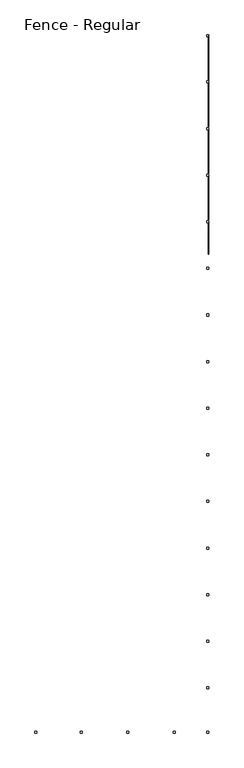
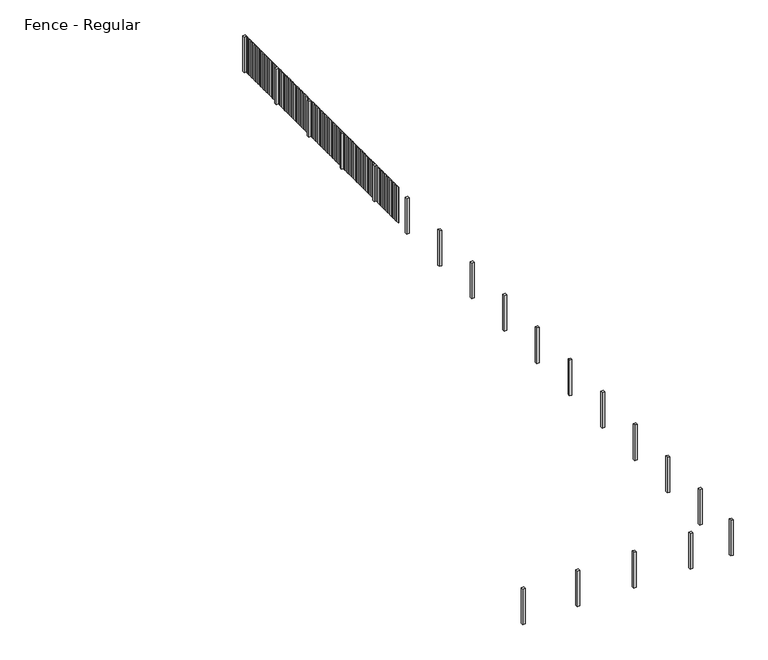
"""IFC4 building model written with IfcOpenShell, lengths in millimetres: railing geometry, Fence - Regular."""

import ifcopenshell
import ifcopenshell.guid

model = None  # the IFC model being written
_history = None  # IfcOwnerHistory: only IFC2X3 demands one
_inside = {}  # id of a spatial element -> (the spatial element, [elements in it])
_under = {}  # id of a project, library or spatial element -> (it, [spatial elements below it])
_declared = {}  # id of a project -> (the project, [libraries it declares])
_typed = {}  # id of a type object -> (the type object, [elements of that type])
_made_of = {}  # id of a material, layer set ... -> (it, [elements and type objects made of it])


def new_model(schema):
    """Start an empty IFC model of exactly this schema.

    Asked for "IFC4X3", IfcOpenShell would pick the latest addendum, in which some entities
    have other attributes; the version numbers below select the first issue.
    IFC2X3 requires an IfcOwnerHistory on every rooted entity: one is made here for all.
    """
    global model, _history
    if schema == "IFC4X3":
        model = ifcopenshell.file(schema_version=(4, 3, 0, 0))
    else:
        model = ifcopenshell.file(schema=schema)
    _inside.clear()
    _under.clear()
    _declared.clear()
    _typed.clear()
    _made_of.clear()
    _history = None
    if model.schema == "IFC2X3":
        org = make("IfcOrganization", Name="unknown")
        user = make(
            "IfcPersonAndOrganization",
            ThePerson=make("IfcPerson", FamilyName="unknown"),
            TheOrganization=org,
        )
        app = make(
            "IfcApplication",
            ApplicationDeveloper=org,
            Version="unknown",
            ApplicationFullName="unknown",
            ApplicationIdentifier="unknown",
        )
        _history = make(
            "IfcOwnerHistory",
            OwningUser=user,
            OwningApplication=app,
            ChangeAction="ADDED",
            CreationDate=0,
        )
    return model


def make(cls, **values):
    """One entity of the class cls with the attributes given. An attribute that is None is left unset."""
    return model.create_entity(
        cls, **{name: value for name, value in values.items() if value is not None}
    )


def rooted(cls, **values):
    """An entity with a GlobalId (a new one), such as an element, a storey or a relation."""
    return make(cls, GlobalId=ifcopenshell.guid.new(), OwnerHistory=_history, **values)


def si_unit(unit_type, name, prefix=None):
    """IfcSIUnit, for example si_unit("LENGTHUNIT", "METRE", prefix="MILLI")."""
    return make("IfcSIUnit", UnitType=unit_type, Prefix=prefix, Name=name)


def assignment(units):
    """IfcUnitAssignment: the units of a project."""
    return None if units is None else make("IfcUnitAssignment", Units=units)


def point(xyz):
    """IfcCartesianPoint."""
    return None if xyz is None else make("IfcCartesianPoint", Coordinates=xyz)


def direction(xyz):
    """IfcDirection."""
    return None if xyz is None else make("IfcDirection", DirectionRatios=xyz)


def frame(location, z_axis=None, x_axis=None):
    """IfcAxis2Placement3D, a coordinate frame: its origin and axes. An axis left out is left unset."""
    return make(
        "IfcAxis2Placement3D",
        Location=point(location),
        Axis=direction(z_axis),
        RefDirection=direction(x_axis),
    )


def origin():
    """The frame at (0, 0, 0) with its axes left unset."""
    return frame((0.0, 0.0, 0.0))


def origin_with_axes():
    """The frame at (0, 0, 0) with the z axis (0, 0, 1) and the x axis (1, 0, 0) written out."""
    return frame((0.0, 0.0, 0.0), z_axis=(0.0, 0.0, 1.0), x_axis=(1.0, 0.0, 0.0))


def place(relative_to, where):
    """IfcLocalPlacement: puts the frame where relative to a parent placement (None: the world)."""
    return make(
        "IfcLocalPlacement", PlacementRelTo=relative_to, RelativePlacement=where
    )


def context(
    kind, dimensions, precision=None, world=None, true_north=None, identifier=None
):
    """IfcGeometricRepresentationContext, for example the 3D "Model" context."""
    return make(
        "IfcGeometricRepresentationContext",
        ContextIdentifier=identifier,
        ContextType=kind,
        CoordinateSpaceDimension=dimensions,
        Precision=precision,
        WorldCoordinateSystem=world,
        TrueNorth=true_north,
    )


def project(units=None, contexts=None):
    """IfcProject with its units and contexts."""
    return rooted(
        "IfcProject",
        Name="project",
        RepresentationContexts=contexts,
        UnitsInContext=assignment(units),
    )


def spatial(cls, under=None, at=None, **own):
    """A site, building, storey or space (cls), placed at a placement, below another one or the project."""
    s = rooted(cls, ObjectPlacement=at, **own)
    if under is not None:
        _under.setdefault(under.id(), (under, []))[1].append(s)
    return s


def polyline(points):
    """IfcPolyline through the points."""
    return make("IfcPolyline", Points=[point(p) for p in points])


def outline(outer, holes=None, kind="AREA"):
    """IfcArbitraryClosedProfileDef: a profile drawn as a closed curve; with holes, ...WithVoids."""
    if holes is None:
        return make("IfcArbitraryClosedProfileDef", ProfileType=kind, OuterCurve=outer)
    return make(
        "IfcArbitraryProfileDefWithVoids",
        ProfileType=kind,
        OuterCurve=outer,
        InnerCurves=holes,
    )


def extrude(swept, where, along, depth):
    """IfcExtrudedAreaSolid: the profile swept, set in the frame where, extruded along a direction by depth."""
    return make(
        "IfcExtrudedAreaSolid",
        SweptArea=swept,
        Position=where,
        ExtrudedDirection=direction(along),
        Depth=depth,
    )


def shape(context_of_items, identifier, shape_type, items):
    """IfcShapeRepresentation: the items that make up one representation, for example the "Body"."""
    return make(
        "IfcShapeRepresentation",
        ContextOfItems=context_of_items,
        RepresentationIdentifier=identifier,
        RepresentationType=shape_type,
        Items=items,
    )


def source(mapping_origin, context_of_items, identifier, shape_type, items):
    """IfcRepresentationMap: a shape defined once, which mapped items show again and again."""
    return make(
        "IfcRepresentationMap",
        MappingOrigin=mapping_origin,
        MappedRepresentation=shape(context_of_items, identifier, shape_type, items),
    )


def transform(
    local_origin,
    x_axis=None,
    y_axis=None,
    z_axis=None,
    scale=None,
    scale2=None,
    scale3=None,
    uniform=True,
):
    """IfcCartesianTransformationOperator3D, or its non-uniform kind. x_axis, y_axis, z_axis: its Axis1, 2, 3."""
    if uniform:
        return make(
            "IfcCartesianTransformationOperator3D",
            Axis1=direction(x_axis),
            Axis2=direction(y_axis),
            LocalOrigin=point(local_origin),
            Scale=scale,
            Axis3=direction(z_axis),
        )
    return make(
        "IfcCartesianTransformationOperator3DnonUniform",
        Axis1=direction(x_axis),
        Axis2=direction(y_axis),
        LocalOrigin=point(local_origin),
        Scale=scale,
        Axis3=direction(z_axis),
        Scale2=scale2,
        Scale3=scale3,
    )


def mapped(mapping_source, mapping_target):
    """IfcMappedItem: shows the shape of a source again, moved by a transform."""
    return make(
        "IfcMappedItem", MappingSource=mapping_source, MappingTarget=mapping_target
    )


def made_of(thing, what):
    """Note that an element or type object is made of a material, layer set ...; save() writes the relation."""
    if what is not None:
        _made_of.setdefault(what.id(), (what, []))[1].append(thing)
    return thing


def element(
    cls,
    number,
    at=None,
    inside=None,
    cuts=None,
    type_object=None,
    material=None,
    context=None,
    identifier="Body",
    shape_type=None,
    held_by="IfcProductDefinitionShape",
    body=None,
    shapes=None,
    **own,
):
    """One element of the class cls, such as IfcWall. Its Tag is "e" and its number.

    at: its placement. inside: the storey or other place that contains it. cuts: it is an
    opening in that element (IfcRelVoidsElement). A single representation is given by context,
    identifier, shape_type and body (its items); several are given by shapes. held_by: the class
    of the entity that holds the representations. save() writes the other relations.
    """
    e = rooted(cls, Tag="e%d" % number, ObjectPlacement=at, **own)
    if body is not None:
        shapes = [shape(context, identifier, shape_type, body)]
    if shapes is not None:
        e.Representation = make(held_by, Representations=shapes)
    if inside is not None:
        _inside.setdefault(inside.id(), (inside, []))[1].append(e)
    if cuts is not None:
        rooted(
            "IfcRelVoidsElement", RelatingBuildingElement=cuts, RelatedOpeningElement=e
        )
    if type_object is not None:
        _typed.setdefault(type_object.id(), (type_object, []))[1].append(e)
    return made_of(e, material)


def aggregate(whole, parts):
    """IfcRelAggregates: a whole, such as a stair, and the parts it consists of."""
    return rooted("IfcRelAggregates", RelatingObject=whole, RelatedObjects=parts)


def save(model, path):
    """Write the relations noted so far, then the file.

    IfcRelAggregates (storeys below a building ...), IfcRelContainedInSpatialStructure (elements
    in a storey), IfcRelDefinesByType, IfcRelAssociatesMaterial and IfcRelDeclares: one each for
    every whole, place, type object, material and project.
    """
    for whole, parts in _under.values():
        aggregate(whole, parts)
    for where, things in _inside.values():
        rooted(
            "IfcRelContainedInSpatialStructure",
            RelatedElements=things,
            RelatingStructure=where,
        )
    for kind, things in _typed.values():
        rooted("IfcRelDefinesByType", RelatedObjects=things, RelatingType=kind)
    for what, things in _made_of.values():
        rooted("IfcRelAssociatesMaterial", RelatedObjects=things, RelatingMaterial=what)
    for by, libraries in _declared.values():
        rooted("IfcRelDeclares", RelatingContext=by, RelatedDefinitions=libraries)
    model.write(path)


def fence_regular_742cfec5(model_context):
    return source(origin(), model_context, "Body", "SweptSolid", [
        extrude(outline(polyline([(34626.2402986, -13051.6917274), (34626.2402986, -13159.6417274), (34607.1902986, -13159.6417274), (34607.1902986, -13051.6917274), (34626.2402986, -13051.6917274)])), origin_with_axes(), (0.0, 0.0, 1.0), 1625.6),
        extrude(outline(polyline([(34626.2402986, -12923.3548853), (34626.2402986, -13031.3048853), (34607.1902986, -13031.3048853), (34607.1902986, -12923.3548853), (34626.2402986, -12923.3548853)])), origin_with_axes(), (0.0, 0.0, 1.0), 1625.6),
        extrude(outline(polyline([(34626.2402986, -12795.0180432), (34626.2402986, -12902.9680432), (34607.1902986, -12902.9680432), (34607.1902986, -12795.0180432), (34626.2402986, -12795.0180432)])), origin_with_axes(), (0.0, 0.0, 1.0), 1625.6),
        extrude(outline(polyline([(34626.2402986, -12666.6812011), (34626.2402986, -12774.6312011), (34607.1902986, -12774.6312011), (34607.1902986, -12666.6812011), (34626.2402986, -12666.6812011)])), origin_with_axes(), (0.0, 0.0, 1.0), 1625.6),
        extrude(outline(polyline([(34626.2402986, -12538.344359), (34626.2402986, -12646.294359), (34607.1902986, -12646.294359), (34607.1902986, -12538.344359), (34626.2402986, -12538.344359)])), origin_with_axes(), (0.0, 0.0, 1.0), 1625.6),
        extrude(outline(polyline([(34626.2402986, -12410.0075169), (34626.2402986, -12517.9575169), (34607.1902986, -12517.9575169), (34607.1902986, -12410.0075169), (34626.2402986, -12410.0075169)])), origin_with_axes(), (0.0, 0.0, 1.0), 1625.6),
        extrude(outline(polyline([(34626.2402986, -12281.6706748), (34626.2402986, -12389.6206748), (34607.1902986, -12389.6206748), (34607.1902986, -12281.6706748), (34626.2402986, -12281.6706748)])), origin_with_axes(), (0.0, 0.0, 1.0), 1625.6),
        extrude(outline(polyline([(34626.2402986, -12153.3338327), (34626.2402986, -12261.2838327), (34607.1902986, -12261.2838327), (34607.1902986, -12153.3338327), (34626.2402986, -12153.3338327)])), origin_with_axes(), (0.0, 0.0, 1.0), 1625.6),
        extrude(outline(polyline([(34626.2402986, -12024.9969906), (34626.2402986, -12132.9469906), (34607.1902986, -12132.9469906), (34607.1902986, -12024.9969906), (34626.2402986, -12024.9969906)])), origin_with_axes(), (0.0, 0.0, 1.0), 1625.6),
        extrude(outline(polyline([(34626.2402986, -11896.6601485), (34626.2402986, -12004.6101485), (34607.1902986, -12004.6101485), (34607.1902986, -11896.6601485), (34626.2402986, -11896.6601485)])), origin_with_axes(), (0.0, 0.0, 1.0), 1625.6),
        extrude(outline(polyline([(34626.2402986, -11768.3233064), (34626.2402986, -11876.2733064), (34607.1902986, -11876.2733064), (34607.1902986, -11768.3233064), (34626.2402986, -11768.3233064)])), origin_with_axes(), (0.0, 0.0, 1.0), 1625.6),
        extrude(outline(polyline([(34626.2402986, -11639.9864643), (34626.2402986, -11747.9364643), (34607.1902986, -11747.9364643), (34607.1902986, -11639.9864643), (34626.2402986, -11639.9864643)])), origin_with_axes(), (0.0, 0.0, 1.0), 1625.6),
        extrude(outline(polyline([(34626.2402986, -11511.6496222), (34626.2402986, -11619.5996222), (34607.1902986, -11619.5996222), (34607.1902986, -11511.6496222), (34626.2402986, -11511.6496222)])), origin_with_axes(), (0.0, 0.0, 1.0), 1625.6),
        extrude(outline(polyline([(34626.2402986, -11254.9759379), (34626.2402986, -11362.9259379), (34607.1902986, -11362.9259379), (34607.1902986, -11254.9759379), (34626.2402986, -11254.9759379)])), origin_with_axes(), (0.0, 0.0, 1.0), 1625.6),
        extrude(outline(polyline([(34626.2402986, -11126.6390958), (34626.2402986, -11234.5890958), (34607.1902986, -11234.5890958), (34607.1902986, -11126.6390958), (34626.2402986, -11126.6390958)])), origin_with_axes(), (0.0, 0.0, 1.0), 1625.6),
        extrude(outline(polyline([(34626.2402986, -10998.3022537), (34626.2402986, -11106.2522537), (34607.1902986, -11106.2522537), (34607.1902986, -10998.3022537), (34626.2402986, -10998.3022537)])), origin_with_axes(), (0.0, 0.0, 1.0), 1625.6),
        extrude(outline(polyline([(34626.2402986, -10869.9654116), (34626.2402986, -10977.9154116), (34607.1902986, -10977.9154116), (34607.1902986, -10869.9654116), (34626.2402986, -10869.9654116)])), origin_with_axes(), (0.0, 0.0, 1.0), 1625.6),
        extrude(outline(polyline([(34626.2402986, -10741.6285695), (34626.2402986, -10849.5785695), (34607.1902986, -10849.5785695), (34607.1902986, -10741.6285695), (34626.2402986, -10741.6285695)])), origin_with_axes(), (0.0, 0.0, 1.0), 1625.6),
        extrude(outline(polyline([(34626.2402986, -10613.2917274), (34626.2402986, -10721.2417274), (34607.1902986, -10721.2417274), (34607.1902986, -10613.2917274), (34626.2402986, -10613.2917274)])), origin_with_axes(), (0.0, 0.0, 1.0), 1625.6),
        extrude(outline(polyline([(34626.2402986, -10484.9548853), (34626.2402986, -10592.9048853), (34607.1902986, -10592.9048853), (34607.1902986, -10484.9548853), (34626.2402986, -10484.9548853)])), origin_with_axes(), (0.0, 0.0, 1.0), 1625.6),
        extrude(outline(polyline([(34626.2402986, -10356.6180432), (34626.2402986, -10464.5680432), (34607.1902986, -10464.5680432), (34607.1902986, -10356.6180432), (34626.2402986, -10356.6180432)])), origin_with_axes(), (0.0, 0.0, 1.0), 1625.6),
        extrude(outline(polyline([(34626.2402986, -10228.2812011), (34626.2402986, -10336.2312011), (34607.1902986, -10336.2312011), (34607.1902986, -10228.2812011), (34626.2402986, -10228.2812011)])), origin_with_axes(), (0.0, 0.0, 1.0), 1625.6),
        extrude(outline(polyline([(34626.2402986, -10099.944359), (34626.2402986, -10207.894359), (34607.1902986, -10207.894359), (34607.1902986, -10099.944359), (34626.2402986, -10099.944359)])), origin_with_axes(), (0.0, 0.0, 1.0), 1625.6),
        extrude(outline(polyline([(34626.2402986, -9971.6075169), (34626.2402986, -10079.5575169), (34607.1902986, -10079.5575169), (34607.1902986, -9971.6075169), (34626.2402986, -9971.6075169)])), origin_with_axes(), (0.0, 0.0, 1.0), 1625.6),
        extrude(outline(polyline([(34626.2402986, -9843.2706748), (34626.2402986, -9951.2206748), (34607.1902986, -9951.2206748), (34607.1902986, -9843.2706748), (34626.2402986, -9843.2706748)])), origin_with_axes(), (0.0, 0.0, 1.0), 1625.6),
        extrude(outline(polyline([(34626.2402986, -9714.9338327), (34626.2402986, -9822.8838327), (34607.1902986, -9822.8838327), (34607.1902986, -9714.9338327), (34626.2402986, -9714.9338327)])), origin_with_axes(), (0.0, 0.0, 1.0), 1625.6),
        extrude(outline(polyline([(34626.2402986, -9586.5969906), (34626.2402986, -9694.5469906), (34607.1902986, -9694.5469906), (34607.1902986, -9586.5969906), (34626.2402986, -9586.5969906)])), origin_with_axes(), (0.0, 0.0, 1.0), 1625.6),
        extrude(outline(polyline([(34626.2402986, -9458.2601485), (34626.2402986, -9566.2101485), (34607.1902986, -9566.2101485), (34607.1902986, -9458.2601485), (34626.2402986, -9458.2601485)])), origin_with_axes(), (0.0, 0.0, 1.0), 1625.6),
        extrude(outline(polyline([(34626.2402986, -9329.9233064), (34626.2402986, -9437.8733064), (34607.1902986, -9437.8733064), (34607.1902986, -9329.9233064), (34626.2402986, -9329.9233064)])), origin_with_axes(), (0.0, 0.0, 1.0), 1625.6),
        extrude(outline(polyline([(34626.2402986, -9201.5864643), (34626.2402986, -9309.5364643), (34607.1902986, -9309.5364643), (34607.1902986, -9201.5864643), (34626.2402986, -9201.5864643)])), origin_with_axes(), (0.0, 0.0, 1.0), 1625.6),
        extrude(outline(polyline([(34626.2402986, -9073.2496222), (34626.2402986, -9181.1996222), (34607.1902986, -9181.1996222), (34607.1902986, -9073.2496222), (34626.2402986, -9073.2496222)])), origin_with_axes(), (0.0, 0.0, 1.0), 1625.6),
        extrude(outline(polyline([(34626.2402986, -8816.5759379), (34626.2402986, -8924.5259379), (34607.1902986, -8924.5259379), (34607.1902986, -8816.5759379), (34626.2402986, -8816.5759379)])), origin_with_axes(), (0.0, 0.0, 1.0), 1625.6),
        extrude(outline(polyline([(34626.2402986, -8688.2390958), (34626.2402986, -8796.1890958), (34607.1902986, -8796.1890958), (34607.1902986, -8688.2390958), (34626.2402986, -8688.2390958)])), origin_with_axes(), (0.0, 0.0, 1.0), 1625.6),
        extrude(outline(polyline([(34626.2402986, -8559.9022537), (34626.2402986, -8667.8522537), (34607.1902986, -8667.8522537), (34607.1902986, -8559.9022537), (34626.2402986, -8559.9022537)])), origin_with_axes(), (0.0, 0.0, 1.0), 1625.6),
        extrude(outline(polyline([(34626.2402986, -8431.5654116), (34626.2402986, -8539.5154116), (34607.1902986, -8539.5154116), (34607.1902986, -8431.5654116), (34626.2402986, -8431.5654116)])), origin_with_axes(), (0.0, 0.0, 1.0), 1625.6),
        extrude(outline(polyline([(34626.2402986, -8303.2285695), (34626.2402986, -8411.1785695), (34607.1902986, -8411.1785695), (34607.1902986, -8303.2285695), (34626.2402986, -8303.2285695)])), origin_with_axes(), (0.0, 0.0, 1.0), 1625.6),
        extrude(outline(polyline([(34626.2402986, -8174.8917274), (34626.2402986, -8282.8417274), (34607.1902986, -8282.8417274), (34607.1902986, -8174.8917274), (34626.2402986, -8174.8917274)])), origin_with_axes(), (0.0, 0.0, 1.0), 1625.6),
        extrude(outline(polyline([(34626.2402986, -8046.5548853), (34626.2402986, -8154.5048853), (34607.1902986, -8154.5048853), (34607.1902986, -8046.5548853), (34626.2402986, -8046.5548853)])), origin_with_axes(), (0.0, 0.0, 1.0), 1625.6),
        extrude(outline(polyline([(34626.2402986, -7918.2180432), (34626.2402986, -8026.1680432), (34607.1902986, -8026.1680432), (34607.1902986, -7918.2180432), (34626.2402986, -7918.2180432)])), origin_with_axes(), (0.0, 0.0, 1.0), 1625.6),
        extrude(outline(polyline([(34626.2402986, -7789.8812011), (34626.2402986, -7897.8312011), (34607.1902986, -7897.8312011), (34607.1902986, -7789.8812011), (34626.2402986, -7789.8812011)])), origin_with_axes(), (0.0, 0.0, 1.0), 1625.6),
        extrude(outline(polyline([(34626.2402986, -7661.544359), (34626.2402986, -7769.494359), (34607.1902986, -7769.494359), (34607.1902986, -7661.544359), (34626.2402986, -7661.544359)])), origin_with_axes(), (0.0, 0.0, 1.0), 1625.6),
        extrude(outline(polyline([(34626.2402986, -7533.2075169), (34626.2402986, -7641.1575169), (34607.1902986, -7641.1575169), (34607.1902986, -7533.2075169), (34626.2402986, -7533.2075169)])), origin_with_axes(), (0.0, 0.0, 1.0), 1625.6),
        extrude(outline(polyline([(34626.2402986, -7404.8706748), (34626.2402986, -7512.8206748), (34607.1902986, -7512.8206748), (34607.1902986, -7404.8706748), (34626.2402986, -7404.8706748)])), origin_with_axes(), (0.0, 0.0, 1.0), 1625.6),
        extrude(outline(polyline([(34626.2402986, -7276.5338327), (34626.2402986, -7384.4838327), (34607.1902986, -7384.4838327), (34607.1902986, -7276.5338327), (34626.2402986, -7276.5338327)])), origin_with_axes(), (0.0, 0.0, 1.0), 1625.6),
        extrude(outline(polyline([(34626.2402986, -7148.1969906), (34626.2402986, -7256.1469906), (34607.1902986, -7256.1469906), (34607.1902986, -7148.1969906), (34626.2402986, -7148.1969906)])), origin_with_axes(), (0.0, 0.0, 1.0), 1625.6),
        extrude(outline(polyline([(34626.2402986, -7019.8601485), (34626.2402986, -7127.8101485), (34607.1902986, -7127.8101485), (34607.1902986, -7019.8601485), (34626.2402986, -7019.8601485)])), origin_with_axes(), (0.0, 0.0, 1.0), 1625.6),
        extrude(outline(polyline([(34626.2402986, -6891.5233064), (34626.2402986, -6999.4733064), (34607.1902986, -6999.4733064), (34607.1902986, -6891.5233064), (34626.2402986, -6891.5233064)])), origin_with_axes(), (0.0, 0.0, 1.0), 1625.6),
        extrude(outline(polyline([(34626.2402986, -6763.1864643), (34626.2402986, -6871.1364643), (34607.1902986, -6871.1364643), (34607.1902986, -6763.1864643), (34626.2402986, -6763.1864643)])), origin_with_axes(), (0.0, 0.0, 1.0), 1625.6),
        extrude(outline(polyline([(34626.2402986, -6634.8496222), (34626.2402986, -6742.7996222), (34607.1902986, -6742.7996222), (34607.1902986, -6634.8496222), (34626.2402986, -6634.8496222)])), origin_with_axes(), (0.0, 0.0, 1.0), 1625.6),
        extrude(outline(polyline([(34626.2402986, -6378.1759379), (34626.2402986, -6486.1259379), (34607.1902986, -6486.1259379), (34607.1902986, -6378.1759379), (34626.2402986, -6378.1759379)])), origin_with_axes(), (0.0, 0.0, 1.0), 1625.6),
        extrude(outline(polyline([(34626.2402986, -6249.8390958), (34626.2402986, -6357.7890958), (34607.1902986, -6357.7890958), (34607.1902986, -6249.8390958), (34626.2402986, -6249.8390958)])), origin_with_axes(), (0.0, 0.0, 1.0), 1625.6),
        extrude(outline(polyline([(34626.2402986, -6121.5022537), (34626.2402986, -6229.4522537), (34607.1902986, -6229.4522537), (34607.1902986, -6121.5022537), (34626.2402986, -6121.5022537)])), origin_with_axes(), (0.0, 0.0, 1.0), 1625.6),
        extrude(outline(polyline([(34626.2402986, -5993.1654116), (34626.2402986, -6101.1154116), (34607.1902986, -6101.1154116), (34607.1902986, -5993.1654116), (34626.2402986, -5993.1654116)])), origin_with_axes(), (0.0, 0.0, 1.0), 1625.6),
        extrude(outline(polyline([(34626.2402986, -5864.8285695), (34626.2402986, -5972.7785695), (34607.1902986, -5972.7785695), (34607.1902986, -5864.8285695), (34626.2402986, -5864.8285695)])), origin_with_axes(), (0.0, 0.0, 1.0), 1625.6),
        extrude(outline(polyline([(34626.2402986, -5736.4917274), (34626.2402986, -5844.4417274), (34607.1902986, -5844.4417274), (34607.1902986, -5736.4917274), (34626.2402986, -5736.4917274)])), origin_with_axes(), (0.0, 0.0, 1.0), 1625.6),
        extrude(outline(polyline([(34626.2402986, -5608.1548853), (34626.2402986, -5716.1048853), (34607.1902986, -5716.1048853), (34607.1902986, -5608.1548853), (34626.2402986, -5608.1548853)])), origin_with_axes(), (0.0, 0.0, 1.0), 1625.6),
        extrude(outline(polyline([(34626.2402986, -5479.8180432), (34626.2402986, -5587.7680432), (34607.1902986, -5587.7680432), (34607.1902986, -5479.8180432), (34626.2402986, -5479.8180432)])), origin_with_axes(), (0.0, 0.0, 1.0), 1625.6),
        extrude(outline(polyline([(34626.2402986, -5351.4812011), (34626.2402986, -5459.4312011), (34607.1902986, -5459.4312011), (34607.1902986, -5351.4812011), (34626.2402986, -5351.4812011)])), origin_with_axes(), (0.0, 0.0, 1.0), 1625.6),
        extrude(outline(polyline([(34626.2402986, -5223.144359), (34626.2402986, -5331.094359), (34607.1902986, -5331.094359), (34607.1902986, -5223.144359), (34626.2402986, -5223.144359)])), origin_with_axes(), (0.0, 0.0, 1.0), 1625.6),
        extrude(outline(polyline([(34626.2402986, -5094.8075169), (34626.2402986, -5202.7575169), (34607.1902986, -5202.7575169), (34607.1902986, -5094.8075169), (34626.2402986, -5094.8075169)])), origin_with_axes(), (0.0, 0.0, 1.0), 1625.6),
        extrude(outline(polyline([(34626.2402986, -4966.4706748), (34626.2402986, -5074.4206748), (34607.1902986, -5074.4206748), (34607.1902986, -4966.4706748), (34626.2402986, -4966.4706748)])), origin_with_axes(), (0.0, 0.0, 1.0), 1625.6),
        extrude(outline(polyline([(34626.2402986, -4838.1338327), (34626.2402986, -4946.0838327), (34607.1902986, -4946.0838327), (34607.1902986, -4838.1338327), (34626.2402986, -4838.1338327)])), origin_with_axes(), (0.0, 0.0, 1.0), 1625.6),
        extrude(outline(polyline([(34626.2402986, -4709.7969906), (34626.2402986, -4817.7469906), (34607.1902986, -4817.7469906), (34607.1902986, -4709.7969906), (34626.2402986, -4709.7969906)])), origin_with_axes(), (0.0, 0.0, 1.0), 1625.6),
        extrude(outline(polyline([(34626.2402986, -4581.4601485), (34626.2402986, -4689.4101485), (34607.1902986, -4689.4101485), (34607.1902986, -4581.4601485), (34626.2402986, -4581.4601485)])), origin_with_axes(), (0.0, 0.0, 1.0), 1625.6),
        extrude(outline(polyline([(34626.2402986, -4453.1233064), (34626.2402986, -4561.0733064), (34607.1902986, -4561.0733064), (34607.1902986, -4453.1233064), (34626.2402986, -4453.1233064)])), origin_with_axes(), (0.0, 0.0, 1.0), 1625.6),
        extrude(outline(polyline([(34626.2402986, -4324.7864643), (34626.2402986, -4432.7364643), (34607.1902986, -4432.7364643), (34607.1902986, -4324.7864643), (34626.2402986, -4324.7864643)])), origin_with_axes(), (0.0, 0.0, 1.0), 1625.6),
        extrude(outline(polyline([(34626.2402986, -4196.4496222), (34626.2402986, -4304.3996222), (34607.1902986, -4304.3996222), (34607.1902986, -4196.4496222), (34626.2402986, -4196.4496222)])), origin_with_axes(), (0.0, 0.0, 1.0), 1625.6),
        extrude(outline(polyline([(34626.2402986, -3939.7759379), (34626.2402986, -4047.7259379), (34607.1902986, -4047.7259379), (34607.1902986, -3939.7759379), (34626.2402986, -3939.7759379)])), origin_with_axes(), (0.0, 0.0, 1.0), 1625.6),
        extrude(outline(polyline([(34626.2402986, -3811.4390958), (34626.2402986, -3919.3890958), (34607.1902986, -3919.3890958), (34607.1902986, -3811.4390958), (34626.2402986, -3811.4390958)])), origin_with_axes(), (0.0, 0.0, 1.0), 1625.6),
        extrude(outline(polyline([(34626.2402986, -3683.1022537), (34626.2402986, -3791.0522537), (34607.1902986, -3791.0522537), (34607.1902986, -3683.1022537), (34626.2402986, -3683.1022537)])), origin_with_axes(), (0.0, 0.0, 1.0), 1625.6),
        extrude(outline(polyline([(34626.2402986, -3554.7654116), (34626.2402986, -3662.7154116), (34607.1902986, -3662.7154116), (34607.1902986, -3554.7654116), (34626.2402986, -3554.7654116)])), origin_with_axes(), (0.0, 0.0, 1.0), 1625.6),
        extrude(outline(polyline([(34626.2402986, -3426.4285695), (34626.2402986, -3534.3785695), (34607.1902986, -3534.3785695), (34607.1902986, -3426.4285695), (34626.2402986, -3426.4285695)])), origin_with_axes(), (0.0, 0.0, 1.0), 1625.6),
        extrude(outline(polyline([(34626.2402986, -3298.0917274), (34626.2402986, -3406.0417274), (34607.1902986, -3406.0417274), (34607.1902986, -3298.0917274), (34626.2402986, -3298.0917274)])), origin_with_axes(), (0.0, 0.0, 1.0), 1625.6),
        extrude(outline(polyline([(34626.2402986, -3169.7548853), (34626.2402986, -3277.7048853), (34607.1902986, -3277.7048853), (34607.1902986, -3169.7548853), (34626.2402986, -3169.7548853)])), origin_with_axes(), (0.0, 0.0, 1.0), 1625.6),
        extrude(outline(polyline([(34626.2402986, -3041.4180432), (34626.2402986, -3149.3680432), (34607.1902986, -3149.3680432), (34607.1902986, -3041.4180432), (34626.2402986, -3041.4180432)])), origin_with_axes(), (0.0, 0.0, 1.0), 1625.6),
        extrude(outline(polyline([(34626.2402986, -2913.0812011), (34626.2402986, -3021.0312011), (34607.1902986, -3021.0312011), (34607.1902986, -2913.0812011), (34626.2402986, -2913.0812011)])), origin_with_axes(), (0.0, 0.0, 1.0), 1625.6),
        extrude(outline(polyline([(34626.2402986, -2784.744359), (34626.2402986, -2892.694359), (34607.1902986, -2892.694359), (34607.1902986, -2784.744359), (34626.2402986, -2784.744359)])), origin_with_axes(), (0.0, 0.0, 1.0), 1625.6),
        extrude(outline(polyline([(34626.2402986, -2656.4075169), (34626.2402986, -2764.3575169), (34607.1902986, -2764.3575169), (34607.1902986, -2656.4075169), (34626.2402986, -2656.4075169)])), origin_with_axes(), (0.0, 0.0, 1.0), 1625.6),
        extrude(outline(polyline([(34626.2402986, -2528.0706748), (34626.2402986, -2636.0206748), (34607.1902986, -2636.0206748), (34607.1902986, -2528.0706748), (34626.2402986, -2528.0706748)])), origin_with_axes(), (0.0, 0.0, 1.0), 1625.6),
        extrude(outline(polyline([(34626.2402986, -2399.7338327), (34626.2402986, -2507.6838327), (34607.1902986, -2507.6838327), (34607.1902986, -2399.7338327), (34626.2402986, -2399.7338327)])), origin_with_axes(), (0.0, 0.0, 1.0), 1625.6),
        extrude(outline(polyline([(34626.2402986, -2271.3969906), (34626.2402986, -2379.3469906), (34607.1902986, -2379.3469906), (34607.1902986, -2271.3969906), (34626.2402986, -2271.3969906)])), origin_with_axes(), (0.0, 0.0, 1.0), 1625.6),
        extrude(outline(polyline([(34626.2402986, -2143.0601485), (34626.2402986, -2251.0101485), (34607.1902986, -2251.0101485), (34607.1902986, -2143.0601485), (34626.2402986, -2143.0601485)])), origin_with_axes(), (0.0, 0.0, 1.0), 1625.6),
        extrude(outline(polyline([(34626.2402986, -2014.7233064), (34626.2402986, -2122.6733064), (34607.1902986, -2122.6733064), (34607.1902986, -2014.7233064), (34626.2402986, -2014.7233064)])), origin_with_axes(), (0.0, 0.0, 1.0), 1625.6),
        extrude(outline(polyline([(34626.2402986, -1886.3864643), (34626.2402986, -1994.3364643), (34607.1902986, -1994.3364643), (34607.1902986, -1886.3864643), (34626.2402986, -1886.3864643)])), origin_with_axes(), (0.0, 0.0, 1.0), 1625.6),
        extrude(outline(polyline([(34626.2402986, -1758.0496222), (34626.2402986, -1865.9996222), (34607.1902986, -1865.9996222), (34607.1902986, -1758.0496222), (34626.2402986, -1758.0496222)])), origin_with_axes(), (0.0, 0.0, 1.0), 1625.6),
        extrude(outline(polyline([(28003.1902986, -38208.88778), (27895.2402986, -38208.88778), (27895.2402986, -38100.93778), (28003.1902986, -38100.93778), (28003.1902986, -38208.88778)])), origin_with_axes(), (0.0, 0.0, 1.0), 1625.6),
        extrude(outline(polyline([(30441.5902986, -38208.88778), (30333.6402986, -38208.88778), (30333.6402986, -38100.93778), (30441.5902986, -38100.93778), (30441.5902986, -38208.88778)])), origin_with_axes(), (0.0, 0.0, 1.0), 1625.6),
        extrude(outline(polyline([(32879.9902986, -38208.88778), (32772.0402986, -38208.88778), (32772.0402986, -38100.93778), (32879.9902986, -38100.93778), (32879.9902986, -38208.88778)])), origin_with_axes(), (0.0, 0.0, 1.0), 1625.6),
        extrude(outline(polyline([(34626.2402986, -38100.93778), (34626.2402986, -38208.88778), (34518.2902986, -38208.88778), (34518.2902986, -38100.93778), (34626.2402986, -38100.93778)])), origin_with_axes(), (0.0, 0.0, 1.0), 1625.6),
        extrude(outline(polyline([(34626.2402986, -35789.53778), (34626.2402986, -35897.48778), (34518.2902986, -35897.48778), (34518.2902986, -35789.53778), (34626.2402986, -35789.53778)])), origin_with_axes(), (0.0, 0.0, 1.0), 1625.6),
        extrude(outline(polyline([(34626.2402986, -33351.13778), (34626.2402986, -33459.08778), (34518.2902986, -33459.08778), (34518.2902986, -33351.13778), (34626.2402986, -33351.13778)])), origin_with_axes(), (0.0, 0.0, 1.0), 1625.6),
        extrude(outline(polyline([(34626.2402986, -30912.73778), (34626.2402986, -31020.68778), (34518.2902986, -31020.68778), (34518.2902986, -30912.73778), (34626.2402986, -30912.73778)])), origin_with_axes(), (0.0, 0.0, 1.0), 1625.6),
        extrude(outline(polyline([(34626.2402986, -28474.33778), (34626.2402986, -28582.28778), (34518.2902986, -28582.28778), (34518.2902986, -28474.33778), (34626.2402986, -28474.33778)])), origin_with_axes(), (0.0, 0.0, 1.0), 1625.6),
        extrude(outline(polyline([(34626.2402986, -26035.93778), (34626.2402986, -26143.88778), (34518.2902986, -26143.88778), (34518.2902986, -26035.93778), (34626.2402986, -26035.93778)])), origin_with_axes(), (0.0, 0.0, 1.0), 1625.6),
        extrude(outline(polyline([(34626.2402986, -23597.53778), (34626.2402986, -23705.48778), (34518.2902986, -23705.48778), (34518.2902986, -23597.53778), (34626.2402986, -23597.53778)])), origin_with_axes(), (0.0, 0.0, 1.0), 1625.6),
        extrude(outline(polyline([(34626.2402986, -21159.13778), (34626.2402986, -21267.08778), (34518.2902986, -21267.08778), (34518.2902986, -21159.13778), (34626.2402986, -21159.13778)])), origin_with_axes(), (0.0, 0.0, 1.0), 1625.6),
        extrude(outline(polyline([(34626.2402986, -18720.73778), (34626.2402986, -18828.68778), (34518.2902986, -18828.68778), (34518.2902986, -18720.73778), (34626.2402986, -18720.73778)])), origin_with_axes(), (0.0, 0.0, 1.0), 1625.6),
        extrude(outline(polyline([(34626.2402986, -16282.33778), (34626.2402986, -16390.28778), (34518.2902986, -16390.28778), (34518.2902986, -16282.33778), (34626.2402986, -16282.33778)])), origin_with_axes(), (0.0, 0.0, 1.0), 1625.6),
        extrude(outline(polyline([(34626.2402986, -13843.93778), (34626.2402986, -13951.88778), (34518.2902986, -13951.88778), (34518.2902986, -13843.93778), (34626.2402986, -13843.93778)])), origin_with_axes(), (0.0, 0.0, 1.0), 1625.6),
        extrude(outline(polyline([(34626.2402986, -11405.53778), (34626.2402986, -11513.48778), (34518.2902986, -11513.48778), (34518.2902986, -11405.53778), (34626.2402986, -11405.53778)])), origin_with_axes(), (0.0, 0.0, 1.0), 1625.6),
        extrude(outline(polyline([(34626.2402986, -8967.13778), (34626.2402986, -9075.08778), (34518.2902986, -9075.08778), (34518.2902986, -8967.13778), (34626.2402986, -8967.13778)])), origin_with_axes(), (0.0, 0.0, 1.0), 1625.6),
        extrude(outline(polyline([(34626.2402986, -6528.73778), (34626.2402986, -6636.68778), (34518.2902986, -6636.68778), (34518.2902986, -6528.73778), (34626.2402986, -6528.73778)])), origin_with_axes(), (0.0, 0.0, 1.0), 1625.6),
        extrude(outline(polyline([(34626.2402986, -4090.33778), (34626.2402986, -4198.28778), (34518.2902986, -4198.28778), (34518.2902986, -4090.33778), (34626.2402986, -4090.33778)])), origin_with_axes(), (0.0, 0.0, 1.0), 1625.6),
        extrude(outline(polyline([(25640.9902986, -38208.88778), (25533.0402986, -38208.88778), (25533.0402986, -38100.93778), (25640.9902986, -38100.93778), (25640.9902986, -38208.88778)])), origin_with_axes(), (0.0, 0.0, 1.0), 1625.6),
        extrude(outline(polyline([(34626.2402986, -1683.68778), (34626.2402986, -1791.63778), (34518.2902986, -1791.63778), (34518.2902986, -1683.68778), (34626.2402986, -1683.68778)])), origin_with_axes(), (0.0, 0.0, 1.0), 1625.6),
    ])


if __name__ == "__main__":
    model = new_model("IFC4")
    model_context = context("Model", 3, world=origin())
    ifc_project = project(units=[si_unit("LENGTHUNIT", "METRE", prefix="MILLI")], contexts=[model_context])
    site = spatial("IfcSite", under=ifc_project)
    building = spatial("IfcBuilding", under=site)
    placement = place(None, origin())
    fence_regular_shape = fence_regular_742cfec5(model_context)
    element("IfcRailing", 1, ObjectType="Fence - Regular", at=placement, inside=building, context=model_context, shape_type="MappedRepresentation", body=[
        mapped(fence_regular_shape, transform((0.0, 0.0, 0.0), x_axis=(1.0, 0.0, 0.0), y_axis=(0.0, 1.0, 0.0), z_axis=(0.0, 0.0, 1.0))),
    ])
    save(model, "model.ifc")

# Revit data of these elements
# Element 1 (IfcRailing, "Fence - Regular")
#   Materials on its faces: "6FT HIGH CEDAR PRIVACY FENCE (SEE DETAIL 3A/A500)"
# Materials
#   "6FT HIGH CEDAR PRIVACY FENCE (SEE DETAIL 3A/A500)": class "Wood", colour RGB 146 120 101, transparency 0, Cost = 0
